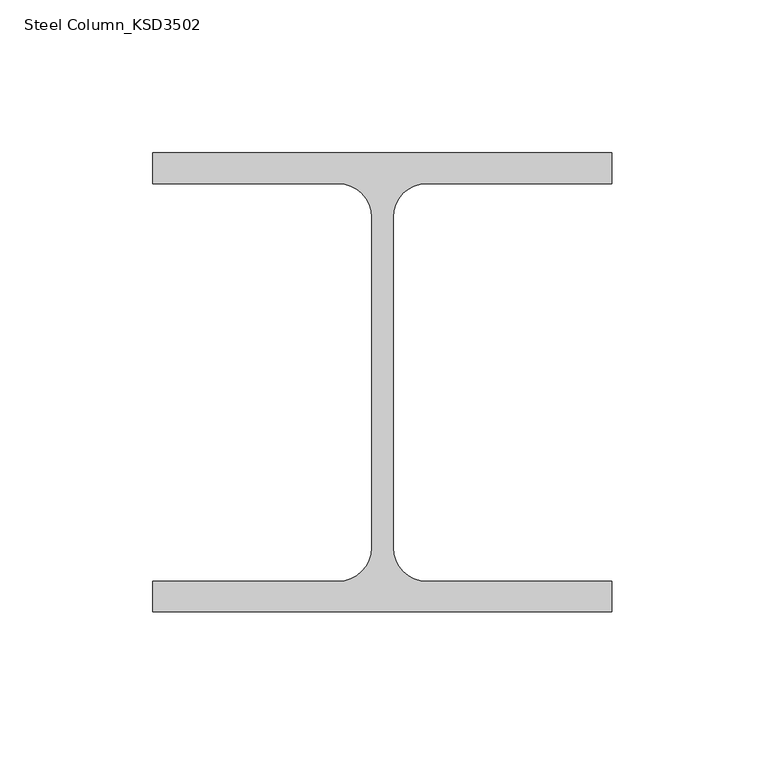
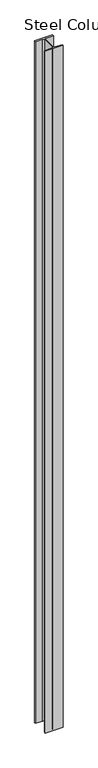
"""IFC4 building model written with IfcOpenShell, lengths in millimetres: column geometry, Steel Column_KSD3502 : H_SC_ASC_H-150×150x7x10."""

import ifcopenshell
import ifcopenshell.guid

model = None  # the IFC model being written
_history = None  # IfcOwnerHistory: only IFC2X3 demands one
_inside = {}  # id of a spatial element -> (the spatial element, [elements in it])
_under = {}  # id of a project, library or spatial element -> (it, [spatial elements below it])
_declared = {}  # id of a project -> (the project, [libraries it declares])
_typed = {}  # id of a type object -> (the type object, [elements of that type])
_made_of = {}  # id of a material, layer set ... -> (it, [elements and type objects made of it])


def new_model(schema):
    """Start an empty IFC model of exactly this schema.

    Asked for "IFC4X3", IfcOpenShell would pick the latest addendum, in which some entities
    have other attributes; the version numbers below select the first issue.
    IFC2X3 requires an IfcOwnerHistory on every rooted entity: one is made here for all.
    """
    global model, _history
    if schema == "IFC4X3":
        model = ifcopenshell.file(schema_version=(4, 3, 0, 0))
    else:
        model = ifcopenshell.file(schema=schema)
    _inside.clear()
    _under.clear()
    _declared.clear()
    _typed.clear()
    _made_of.clear()
    _history = None
    if model.schema == "IFC2X3":
        org = make("IfcOrganization", Name="unknown")
        user = make(
            "IfcPersonAndOrganization",
            ThePerson=make("IfcPerson", FamilyName="unknown"),
            TheOrganization=org,
        )
        app = make(
            "IfcApplication",
            ApplicationDeveloper=org,
            Version="unknown",
            ApplicationFullName="unknown",
            ApplicationIdentifier="unknown",
        )
        _history = make(
            "IfcOwnerHistory",
            OwningUser=user,
            OwningApplication=app,
            ChangeAction="ADDED",
            CreationDate=0,
        )
    return model


def make(cls, **values):
    """One entity of the class cls with the attributes given. An attribute that is None is left unset."""
    return model.create_entity(
        cls, **{name: value for name, value in values.items() if value is not None}
    )


def rooted(cls, **values):
    """An entity with a GlobalId (a new one), such as an element, a storey or a relation."""
    return make(cls, GlobalId=ifcopenshell.guid.new(), OwnerHistory=_history, **values)


def si_unit(unit_type, name, prefix=None):
    """IfcSIUnit, for example si_unit("LENGTHUNIT", "METRE", prefix="MILLI")."""
    return make("IfcSIUnit", UnitType=unit_type, Prefix=prefix, Name=name)


def assignment(units):
    """IfcUnitAssignment: the units of a project."""
    return None if units is None else make("IfcUnitAssignment", Units=units)


def point(xyz):
    """IfcCartesianPoint."""
    return None if xyz is None else make("IfcCartesianPoint", Coordinates=xyz)


def direction(xyz):
    """IfcDirection."""
    return None if xyz is None else make("IfcDirection", DirectionRatios=xyz)


def frame(location, z_axis=None, x_axis=None):
    """IfcAxis2Placement3D, a coordinate frame: its origin and axes. An axis left out is left unset."""
    return make(
        "IfcAxis2Placement3D",
        Location=point(location),
        Axis=direction(z_axis),
        RefDirection=direction(x_axis),
    )


def frame_2d(location, x_axis=None):
    """IfcAxis2Placement2D, a coordinate frame in the plane: its origin and x axis."""
    return make(
        "IfcAxis2Placement2D", Location=point(location), RefDirection=direction(x_axis)
    )


def origin():
    """The frame at (0, 0, 0) with its axes left unset."""
    return frame((0.0, 0.0, 0.0))


def place(relative_to, where):
    """IfcLocalPlacement: puts the frame where relative to a parent placement (None: the world)."""
    return make(
        "IfcLocalPlacement", PlacementRelTo=relative_to, RelativePlacement=where
    )


def context(
    kind, dimensions, precision=None, world=None, true_north=None, identifier=None
):
    """IfcGeometricRepresentationContext, for example the 3D "Model" context."""
    return make(
        "IfcGeometricRepresentationContext",
        ContextIdentifier=identifier,
        ContextType=kind,
        CoordinateSpaceDimension=dimensions,
        Precision=precision,
        WorldCoordinateSystem=world,
        TrueNorth=true_north,
    )


def project(units=None, contexts=None):
    """IfcProject with its units and contexts."""
    return rooted(
        "IfcProject",
        Name="project",
        RepresentationContexts=contexts,
        UnitsInContext=assignment(units),
    )


def spatial(cls, under=None, at=None, **own):
    """A site, building, storey or space (cls), placed at a placement, below another one or the project."""
    s = rooted(cls, ObjectPlacement=at, **own)
    if under is not None:
        _under.setdefault(under.id(), (under, []))[1].append(s)
    return s


def polyline(points):
    """IfcPolyline through the points."""
    return make("IfcPolyline", Points=[point(p) for p in points])


def circle_curve(where, radius):
    """IfcCircle in the frame where."""
    return make("IfcCircle", Position=where, Radius=radius)


def trimmed(basis, trim1, trim2, sense, master):
    """IfcTrimmedCurve: the piece of a basis curve between two trims."""
    return make(
        "IfcTrimmedCurve",
        BasisCurve=basis,
        Trim1=trim1,
        Trim2=trim2,
        SenseAgreement=sense,
        MasterRepresentation=master,
    )


def segment(curve, same_sense, transition):
    """IfcCompositeCurveSegment."""
    return make(
        "IfcCompositeCurveSegment",
        Transition=transition,
        SameSense=same_sense,
        ParentCurve=curve,
    )


def composite_curve(segments, self_intersect=None):
    """IfcCompositeCurve: segments joined end to end."""
    return make("IfcCompositeCurve", Segments=segments, SelfIntersect=self_intersect)


def outline(outer, holes=None, kind="AREA"):
    """IfcArbitraryClosedProfileDef: a profile drawn as a closed curve; with holes, ...WithVoids."""
    if holes is None:
        return make("IfcArbitraryClosedProfileDef", ProfileType=kind, OuterCurve=outer)
    return make(
        "IfcArbitraryProfileDefWithVoids",
        ProfileType=kind,
        OuterCurve=outer,
        InnerCurves=holes,
    )


def extrude(swept, where, along, depth):
    """IfcExtrudedAreaSolid: the profile swept, set in the frame where, extruded along a direction by depth."""
    return make(
        "IfcExtrudedAreaSolid",
        SweptArea=swept,
        Position=where,
        ExtrudedDirection=direction(along),
        Depth=depth,
    )


def shape(context_of_items, identifier, shape_type, items):
    """IfcShapeRepresentation: the items that make up one representation, for example the "Body"."""
    return make(
        "IfcShapeRepresentation",
        ContextOfItems=context_of_items,
        RepresentationIdentifier=identifier,
        RepresentationType=shape_type,
        Items=items,
    )


def source(mapping_origin, context_of_items, identifier, shape_type, items):
    """IfcRepresentationMap: a shape defined once, which mapped items show again and again."""
    return make(
        "IfcRepresentationMap",
        MappingOrigin=mapping_origin,
        MappedRepresentation=shape(context_of_items, identifier, shape_type, items),
    )


def transform(
    local_origin,
    x_axis=None,
    y_axis=None,
    z_axis=None,
    scale=None,
    scale2=None,
    scale3=None,
    uniform=True,
):
    """IfcCartesianTransformationOperator3D, or its non-uniform kind. x_axis, y_axis, z_axis: its Axis1, 2, 3."""
    if uniform:
        return make(
            "IfcCartesianTransformationOperator3D",
            Axis1=direction(x_axis),
            Axis2=direction(y_axis),
            LocalOrigin=point(local_origin),
            Scale=scale,
            Axis3=direction(z_axis),
        )
    return make(
        "IfcCartesianTransformationOperator3DnonUniform",
        Axis1=direction(x_axis),
        Axis2=direction(y_axis),
        LocalOrigin=point(local_origin),
        Scale=scale,
        Axis3=direction(z_axis),
        Scale2=scale2,
        Scale3=scale3,
    )


def mapped(mapping_source, mapping_target):
    """IfcMappedItem: shows the shape of a source again, moved by a transform."""
    return make(
        "IfcMappedItem", MappingSource=mapping_source, MappingTarget=mapping_target
    )


def made_of(thing, what):
    """Note that an element or type object is made of a material, layer set ...; save() writes the relation."""
    if what is not None:
        _made_of.setdefault(what.id(), (what, []))[1].append(thing)
    return thing


def element(
    cls,
    number,
    at=None,
    inside=None,
    cuts=None,
    type_object=None,
    material=None,
    context=None,
    identifier="Body",
    shape_type=None,
    held_by="IfcProductDefinitionShape",
    body=None,
    shapes=None,
    **own,
):
    """One element of the class cls, such as IfcWall. Its Tag is "e" and its number.

    at: its placement. inside: the storey or other place that contains it. cuts: it is an
    opening in that element (IfcRelVoidsElement). A single representation is given by context,
    identifier, shape_type and body (its items); several are given by shapes. held_by: the class
    of the entity that holds the representations. save() writes the other relations.
    """
    e = rooted(cls, Tag="e%d" % number, ObjectPlacement=at, **own)
    if body is not None:
        shapes = [shape(context, identifier, shape_type, body)]
    if shapes is not None:
        e.Representation = make(held_by, Representations=shapes)
    if inside is not None:
        _inside.setdefault(inside.id(), (inside, []))[1].append(e)
    if cuts is not None:
        rooted(
            "IfcRelVoidsElement", RelatingBuildingElement=cuts, RelatedOpeningElement=e
        )
    if type_object is not None:
        _typed.setdefault(type_object.id(), (type_object, []))[1].append(e)
    return made_of(e, material)


def aggregate(whole, parts):
    """IfcRelAggregates: a whole, such as a stair, and the parts it consists of."""
    return rooted("IfcRelAggregates", RelatingObject=whole, RelatedObjects=parts)


def save(model, path):
    """Write the relations noted so far, then the file.

    IfcRelAggregates (storeys below a building ...), IfcRelContainedInSpatialStructure (elements
    in a storey), IfcRelDefinesByType, IfcRelAssociatesMaterial and IfcRelDeclares: one each for
    every whole, place, type object, material and project.
    """
    for whole, parts in _under.values():
        aggregate(whole, parts)
    for where, things in _inside.values():
        rooted(
            "IfcRelContainedInSpatialStructure",
            RelatedElements=things,
            RelatingStructure=where,
        )
    for kind, things in _typed.values():
        rooted("IfcRelDefinesByType", RelatedObjects=things, RelatingType=kind)
    for what, things in _made_of.values():
        rooted("IfcRelAssociatesMaterial", RelatedObjects=things, RelatingMaterial=what)
    for by, libraries in _declared.values():
        rooted("IfcRelDeclares", RelatingContext=by, RelatedDefinitions=libraries)
    model.write(path)


def steel_column_ksd3502_5fc823e1(model_context):
    return source(origin(), model_context, "Body", "SweptSolid", [
        extrude(outline(composite_curve([segment(polyline([(75.0, 75.0), (75.0, 65.0), (14.5, 65.0)]), True, "CONTINUOUS"), segment(trimmed(circle_curve(frame_2d((14.5, 54.0)), 11.0), [point((14.5, 65.0))], [point((3.5, 54.0))], True, "CARTESIAN"), True, "CONTINUOUS"), segment(polyline([(3.5, 54.0), (3.5, -54.0)]), True, "CONTINUOUS"), segment(trimmed(circle_curve(frame_2d((14.5, -54.0)), 11.0), [point((3.5, -54.0))], [point((14.5, -65.0))], True, "CARTESIAN"), True, "CONTINUOUS"), segment(polyline([(14.5, -65.0), (75.0, -65.0), (75.0, -75.0), (-75.0, -75.0), (-75.0, -65.0), (-14.5, -65.0)]), True, "CONTINUOUS"), segment(trimmed(circle_curve(frame_2d((-14.5, -54.0)), 11.0), [point((-14.5, -65.0))], [point((-3.5, -54.0))], True, "CARTESIAN"), True, "CONTINUOUS"), segment(polyline([(-3.5, -54.0), (-3.5, 54.0)]), True, "CONTINUOUS"), segment(trimmed(circle_curve(frame_2d((-14.5, 54.0)), 11.0), [point((-3.5, 54.0))], [point((-14.5, 65.0))], True, "CARTESIAN"), True, "CONTINUOUS"), segment(polyline([(-14.5, 65.0), (-75.0, 65.0), (-75.0, 75.0), (75.0, 75.0)]), True, "CONTINUOUS")], self_intersect=False)), frame((0.0, 0.0, 599.9720055), z_axis=(0.0, 0.0, 1.0), x_axis=(1.0, 0.0, 0.0)), (0.0, 0.0, 1.0), 6000.0),
    ])


if __name__ == "__main__":
    model = new_model("IFC4")
    model_context = context("Model", 3, world=origin())
    ifc_project = project(units=[si_unit("LENGTHUNIT", "METRE", prefix="MILLI")], contexts=[model_context])
    site = spatial("IfcSite", under=ifc_project)
    building = spatial("IfcBuilding", under=site)
    placement = place(None, origin())
    steel_column_ksd3502_shape = steel_column_ksd3502_5fc823e1(model_context)
    element("IfcColumn", 1, ObjectType="Steel Column_KSD3502 : H_SC_ASC_H-150×150x7x10", at=placement, inside=building, context=model_context, shape_type="MappedRepresentation", body=[
        mapped(steel_column_ksd3502_shape, transform((0.0, 0.0, 0.0), x_axis=(1.0, 0.0, 0.0), y_axis=(0.0, 1.0, 0.0), z_axis=(0.0, 0.0, 1.0))),
    ])
    save(model, "model.ifc")

# Revit data of these elements
# Type "Steel Column_KSD3502 : H_SC_ASC_H-150×150x7x10"
#   Width = 15.0 cm
#   Web Thickness = 0.7 cm
#   Web Fillet = 1.1 cm
#   Warping Constant = 27562.5 cm⁶
#   Torsional Moment of Inertia = 11.6007 cm⁴
#   Section Area = 40.14 cm²
#   Plastic Modulus weak axis = 115.0 cm³
#   Plastic Modulus strong axis = 246.0 cm³
#   Perimeter = 1.27 m²/m
#   Nominal Weight = 31.50 kgf/m
#   Moment of Inertia weak axis = 563.00 cm⁴
#   Moment of Inertia strong axis = 1640.00 cm⁴
#   Height = 15.0 cm
#   Flange Thickness = 1.0 cm
#   Elastic Modulus weak axis = 75.1 cm³
#   Elastic Modulus strong axis = 219.0 cm³
#   Centroid Vertical = 7.5 cm
#   Centroid Horizontal = 7.5 cm
#   Bolt Spacing = 13.97 cm
#   Structural Material [instance default] = Steel, 45-345
#   Section Name Key = ""
#   Assembly Code = ""
# Element 1 (IfcColumn, "Steel Column_KSD3502 : H_SC_ASC_H-150×150x7x10")
#   Structural Material = A03AD029-00005_Anchor Bolt (Installation only)_M24
#   Materials on its faces: "A03AD029-00005_Anchor Bolt (Installation only)_M24"
# Materials
#   "Steel, 45-345": class "Metal", colour RGB 189 187 185, transparency 0, Description = "Steel 345 MPa", Cost = 0
#   "A03AD029-00005_Anchor Bolt (Installation only)_M24": class "Unassigned", colour RGB 84 83 81, transparency 0, Cost = 0
